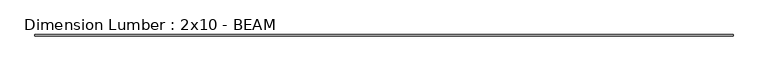
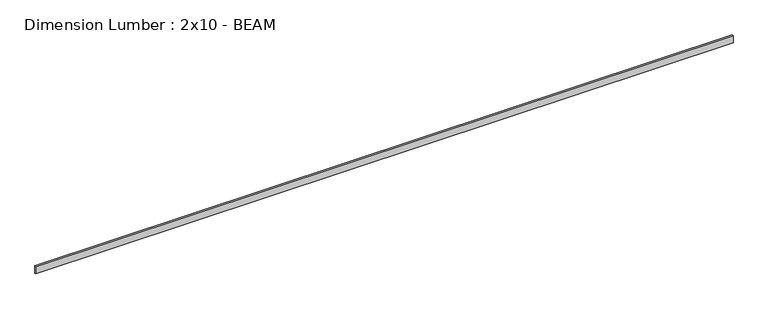
"""IFC4 building model written with IfcOpenShell, lengths in millimetres: beam geometry, Dimension Lumber : 2x10 - BEAM."""

from ifc_helpers import new_model, si_unit, frame, origin, place, context, project, spatial, polyline, outline, extrude, source, transform, mapped, element, save


def dimension_lumber_2x10_beam_ea8148c9(model_context):
    return source(origin(), model_context, "Body", "SweptSolid", [
        extrude(outline(polyline([(10486.8725685, 19.05), (10486.8725685, -19.05), (-10790.3899315, -19.05), (-10790.3899315, 19.05), (10486.8725685, 19.05)])), frame((0.0, 0.0, -117.475), z_axis=(0.0, 0.0, 1.0), x_axis=(1.0, 0.0, 0.0)), (0.0, 0.0, 1.0), 234.95),
    ])


if __name__ == "__main__":
    model = new_model("IFC4")
    model_context = context("Model", 3, world=origin())
    ifc_project = project(units=[si_unit("LENGTHUNIT", "METRE", prefix="MILLI")], contexts=[model_context])
    site = spatial("IfcSite", under=ifc_project)
    building = spatial("IfcBuilding", under=site)
    placement = place(None, origin())
    dimension_lumber_2x10_beam_shape = dimension_lumber_2x10_beam_ea8148c9(model_context)
    element("IfcBeam", 1, ObjectType="Dimension Lumber : 2x10 - BEAM", at=placement, inside=building, context=model_context, shape_type="MappedRepresentation", body=[
        mapped(dimension_lumber_2x10_beam_shape, transform((0.0, 0.0, 0.0), x_axis=(1.0, 0.0, 0.0), y_axis=(0.0, 1.0, 0.0), z_axis=(0.0, 0.0, 1.0))),
    ])
    save(model, "model.ifc")

# Revit data of these elements
# Type "Dimension Lumber : 2x10 - BEAM"
#   Assembly Code = "B10"
#   A = 0.0755556 SF
#   Length [instance default] = 5' - 0"
#   b = 0' - 1 1/2"
#   d = 0' - 9 1/4"
#   Structural Material = (3) SISTERED 2X10s AT BEAM
# Element 1 (IfcBeam, "Dimension Lumber : 2x10 - BEAM")
#   Materials on its faces: "(3) SISTERED 2X10s AT BEAM"
# Materials
#   "(3) SISTERED 2X10s AT BEAM": class "Wood", colour RGB 234 198 147, transparency 0, Description = "Pinus Echinata", Cost = 0
